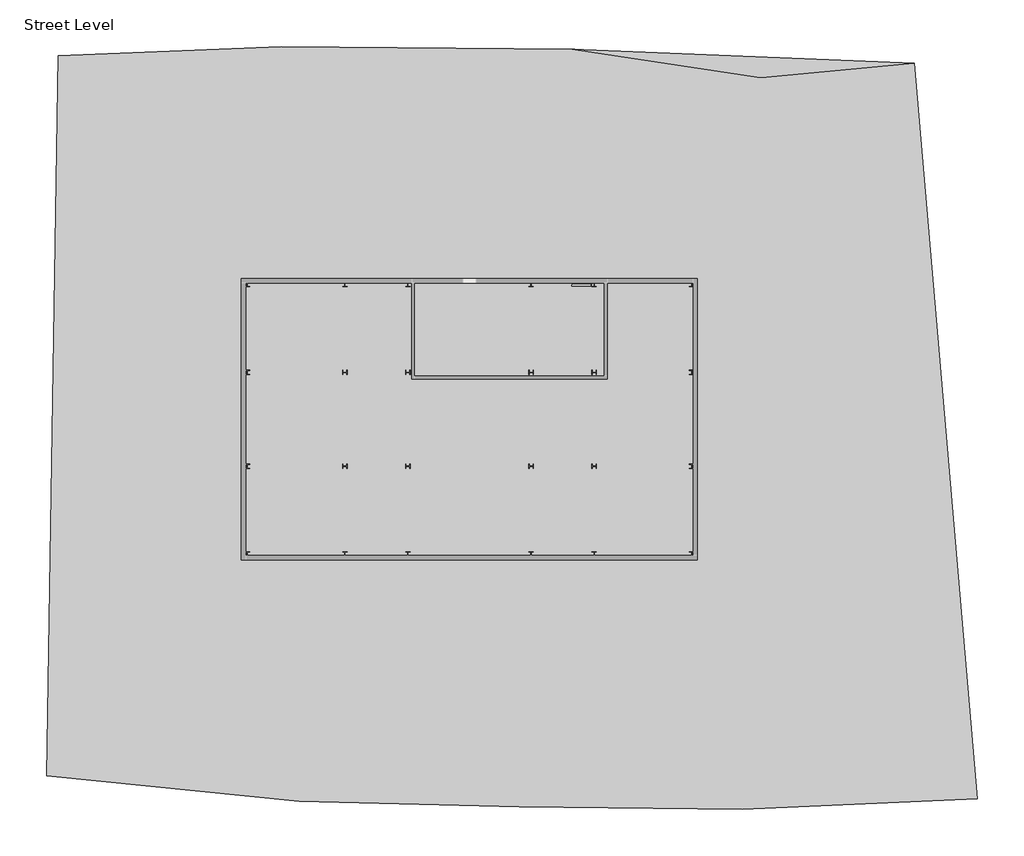
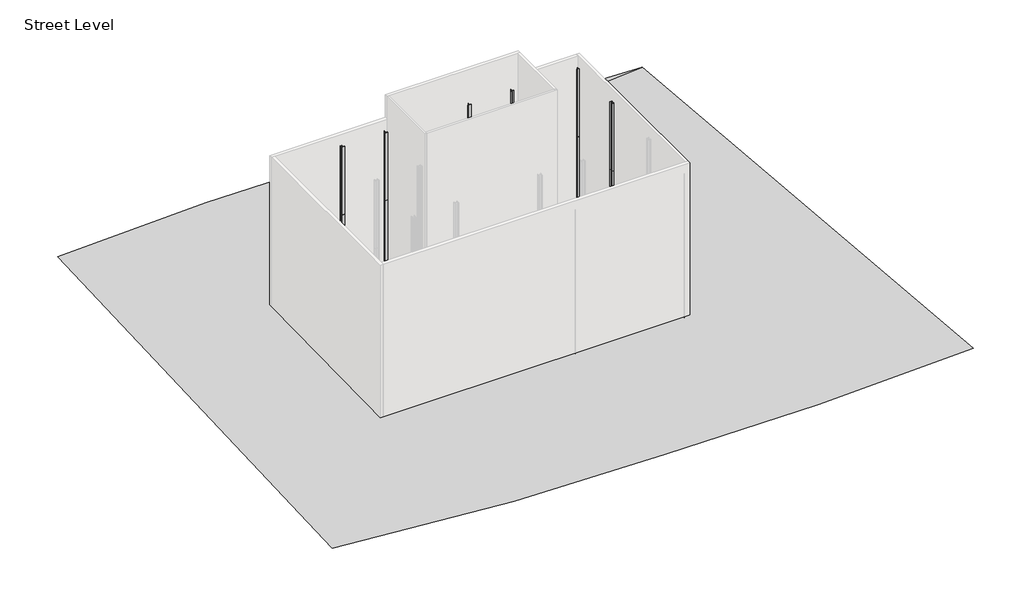
# One storey, part 3 of 3: 8 columns, 1 member, 1 proxy.
"""IFC4 building model written with IfcOpenShell, lengths in millimetres."""

import ifcopenshell
import ifcopenshell.guid

model = None  # the IFC model being written
_history = None  # IfcOwnerHistory: only IFC2X3 demands one
_inside = {}  # id of a spatial element -> (the spatial element, [elements in it])
_under = {}  # id of a project, library or spatial element -> (it, [spatial elements below it])
_declared = {}  # id of a project -> (the project, [libraries it declares])
_typed = {}  # id of a type object -> (the type object, [elements of that type])
_made_of = {}  # id of a material, layer set ... -> (it, [elements and type objects made of it])


def new_model(schema):
    """Start an empty IFC model of exactly this schema.

    Asked for "IFC4X3", IfcOpenShell would pick the latest addendum, in which some entities
    have other attributes; the version numbers below select the first issue.
    IFC2X3 requires an IfcOwnerHistory on every rooted entity: one is made here for all.
    """
    global model, _history
    if schema == "IFC4X3":
        model = ifcopenshell.file(schema_version=(4, 3, 0, 0))
    else:
        model = ifcopenshell.file(schema=schema)
    _inside.clear()
    _under.clear()
    _declared.clear()
    _typed.clear()
    _made_of.clear()
    _history = None
    if model.schema == "IFC2X3":
        org = make("IfcOrganization", Name="unknown")
        user = make(
            "IfcPersonAndOrganization",
            ThePerson=make("IfcPerson", FamilyName="unknown"),
            TheOrganization=org,
        )
        app = make(
            "IfcApplication",
            ApplicationDeveloper=org,
            Version="unknown",
            ApplicationFullName="unknown",
            ApplicationIdentifier="unknown",
        )
        _history = make(
            "IfcOwnerHistory",
            OwningUser=user,
            OwningApplication=app,
            ChangeAction="ADDED",
            CreationDate=0,
        )
    return model


def make(cls, **values):
    """One entity of the class cls with the attributes given. An attribute that is None is left unset."""
    return model.create_entity(
        cls, **{name: value for name, value in values.items() if value is not None}
    )


def rooted(cls, **values):
    """An entity with a GlobalId (a new one), such as an element, a storey or a relation."""
    return make(cls, GlobalId=ifcopenshell.guid.new(), OwnerHistory=_history, **values)


def si_unit(unit_type, name, prefix=None):
    """IfcSIUnit, for example si_unit("LENGTHUNIT", "METRE", prefix="MILLI")."""
    return make("IfcSIUnit", UnitType=unit_type, Prefix=prefix, Name=name)


def assignment(units):
    """IfcUnitAssignment: the units of a project."""
    return None if units is None else make("IfcUnitAssignment", Units=units)


def point(xyz):
    """IfcCartesianPoint."""
    return None if xyz is None else make("IfcCartesianPoint", Coordinates=xyz)


def direction(xyz):
    """IfcDirection."""
    return None if xyz is None else make("IfcDirection", DirectionRatios=xyz)


def frame(location, z_axis=None, x_axis=None):
    """IfcAxis2Placement3D, a coordinate frame: its origin and axes. An axis left out is left unset."""
    return make(
        "IfcAxis2Placement3D",
        Location=point(location),
        Axis=direction(z_axis),
        RefDirection=direction(x_axis),
    )


def frame_2d(location, x_axis=None):
    """IfcAxis2Placement2D, a coordinate frame in the plane: its origin and x axis."""
    return make(
        "IfcAxis2Placement2D", Location=point(location), RefDirection=direction(x_axis)
    )


def origin():
    """The frame at (0, 0, 0) with its axes left unset."""
    return frame((0.0, 0.0, 0.0))


def place(relative_to, where):
    """IfcLocalPlacement: puts the frame where relative to a parent placement (None: the world)."""
    return make(
        "IfcLocalPlacement", PlacementRelTo=relative_to, RelativePlacement=where
    )


def context(
    kind, dimensions, precision=None, world=None, true_north=None, identifier=None
):
    """IfcGeometricRepresentationContext, for example the 3D "Model" context."""
    return make(
        "IfcGeometricRepresentationContext",
        ContextIdentifier=identifier,
        ContextType=kind,
        CoordinateSpaceDimension=dimensions,
        Precision=precision,
        WorldCoordinateSystem=world,
        TrueNorth=true_north,
    )


def project(units=None, contexts=None):
    """IfcProject with its units and contexts."""
    return rooted(
        "IfcProject",
        Name="project",
        RepresentationContexts=contexts,
        UnitsInContext=assignment(units),
    )


def spatial(cls, under=None, at=None, **own):
    """A site, building, storey or space (cls), placed at a placement, below another one or the project."""
    s = rooted(cls, ObjectPlacement=at, **own)
    if under is not None:
        _under.setdefault(under.id(), (under, []))[1].append(s)
    return s


def polyline(points):
    """IfcPolyline through the points."""
    return make("IfcPolyline", Points=[point(p) for p in points])


def point_list(points):
    """IfcCartesianPointList2D or 3D."""
    cls = (
        "IfcCartesianPointList2D" if len(points[0]) == 2 else "IfcCartesianPointList3D"
    )
    return make(cls, CoordList=points)


def circle_curve(where, radius):
    """IfcCircle in the frame where."""
    return make("IfcCircle", Position=where, Radius=radius)


def trimmed(basis, trim1, trim2, sense, master):
    """IfcTrimmedCurve: the piece of a basis curve between two trims."""
    return make(
        "IfcTrimmedCurve",
        BasisCurve=basis,
        Trim1=trim1,
        Trim2=trim2,
        SenseAgreement=sense,
        MasterRepresentation=master,
    )


def segment(curve, same_sense, transition):
    """IfcCompositeCurveSegment."""
    return make(
        "IfcCompositeCurveSegment",
        Transition=transition,
        SameSense=same_sense,
        ParentCurve=curve,
    )


def composite_curve(segments, self_intersect=None):
    """IfcCompositeCurve: segments joined end to end."""
    return make("IfcCompositeCurve", Segments=segments, SelfIntersect=self_intersect)


def outline(outer, holes=None, kind="AREA"):
    """IfcArbitraryClosedProfileDef: a profile drawn as a closed curve; with holes, ...WithVoids."""
    if holes is None:
        return make("IfcArbitraryClosedProfileDef", ProfileType=kind, OuterCurve=outer)
    return make(
        "IfcArbitraryProfileDefWithVoids",
        ProfileType=kind,
        OuterCurve=outer,
        InnerCurves=holes,
    )


def extrude(swept, where, along, depth):
    """IfcExtrudedAreaSolid: the profile swept, set in the frame where, extruded along a direction by depth."""
    return make(
        "IfcExtrudedAreaSolid",
        SweptArea=swept,
        Position=where,
        ExtrudedDirection=direction(along),
        Depth=depth,
    )


def triangles(points, corners, closed=None, point_numbers=None):
    """IfcTriangulatedFaceSet: each triangle names its three corners, points numbered from 1."""
    return make(
        "IfcTriangulatedFaceSet",
        Coordinates=point_list(points),
        Closed=closed,
        CoordIndex=corners,
        PnIndex=point_numbers,
    )


def shape(context_of_items, identifier, shape_type, items):
    """IfcShapeRepresentation: the items that make up one representation, for example the "Body"."""
    return make(
        "IfcShapeRepresentation",
        ContextOfItems=context_of_items,
        RepresentationIdentifier=identifier,
        RepresentationType=shape_type,
        Items=items,
    )


def source(mapping_origin, context_of_items, identifier, shape_type, items):
    """IfcRepresentationMap: a shape defined once, which mapped items show again and again."""
    return make(
        "IfcRepresentationMap",
        MappingOrigin=mapping_origin,
        MappedRepresentation=shape(context_of_items, identifier, shape_type, items),
    )


def transform(
    local_origin,
    x_axis=None,
    y_axis=None,
    z_axis=None,
    scale=None,
    scale2=None,
    scale3=None,
    uniform=True,
):
    """IfcCartesianTransformationOperator3D, or its non-uniform kind. x_axis, y_axis, z_axis: its Axis1, 2, 3."""
    if uniform:
        return make(
            "IfcCartesianTransformationOperator3D",
            Axis1=direction(x_axis),
            Axis2=direction(y_axis),
            LocalOrigin=point(local_origin),
            Scale=scale,
            Axis3=direction(z_axis),
        )
    return make(
        "IfcCartesianTransformationOperator3DnonUniform",
        Axis1=direction(x_axis),
        Axis2=direction(y_axis),
        LocalOrigin=point(local_origin),
        Scale=scale,
        Axis3=direction(z_axis),
        Scale2=scale2,
        Scale3=scale3,
    )


def mapped(mapping_source, mapping_target):
    """IfcMappedItem: shows the shape of a source again, moved by a transform."""
    return make(
        "IfcMappedItem", MappingSource=mapping_source, MappingTarget=mapping_target
    )


def made_of(thing, what):
    """Note that an element or type object is made of a material, layer set ...; save() writes the relation."""
    if what is not None:
        _made_of.setdefault(what.id(), (what, []))[1].append(thing)
    return thing


def element(
    cls,
    number,
    at=None,
    inside=None,
    cuts=None,
    type_object=None,
    material=None,
    context=None,
    identifier="Body",
    shape_type=None,
    held_by="IfcProductDefinitionShape",
    body=None,
    shapes=None,
    **own,
):
    """One element of the class cls, such as IfcWall. Its Tag is "e" and its number.

    at: its placement. inside: the storey or other place that contains it. cuts: it is an
    opening in that element (IfcRelVoidsElement). A single representation is given by context,
    identifier, shape_type and body (its items); several are given by shapes. held_by: the class
    of the entity that holds the representations. save() writes the other relations.
    """
    e = rooted(cls, Tag="e%d" % number, ObjectPlacement=at, **own)
    if body is not None:
        shapes = [shape(context, identifier, shape_type, body)]
    if shapes is not None:
        e.Representation = make(held_by, Representations=shapes)
    if inside is not None:
        _inside.setdefault(inside.id(), (inside, []))[1].append(e)
    if cuts is not None:
        rooted(
            "IfcRelVoidsElement", RelatingBuildingElement=cuts, RelatedOpeningElement=e
        )
    if type_object is not None:
        _typed.setdefault(type_object.id(), (type_object, []))[1].append(e)
    return made_of(e, material)


def aggregate(whole, parts):
    """IfcRelAggregates: a whole, such as a stair, and the parts it consists of."""
    return rooted("IfcRelAggregates", RelatingObject=whole, RelatedObjects=parts)


def save(model, path):
    """Write the relations noted so far, then the file.

    IfcRelAggregates (storeys below a building ...), IfcRelContainedInSpatialStructure (elements
    in a storey), IfcRelDefinesByType, IfcRelAssociatesMaterial and IfcRelDeclares: one each for
    every whole, place, type object, material and project.
    """
    for whole, parts in _under.values():
        aggregate(whole, parts)
    for where, things in _inside.values():
        rooted(
            "IfcRelContainedInSpatialStructure",
            RelatedElements=things,
            RelatingStructure=where,
        )
    for kind, things in _typed.values():
        rooted("IfcRelDefinesByType", RelatedObjects=things, RelatingType=kind)
    for what, things in _made_of.values():
        rooted("IfcRelAssociatesMaterial", RelatedObjects=things, RelatingMaterial=what)
    for by, libraries in _declared.values():
        rooted("IfcRelDeclares", RelatingContext=by, RelatedDefinitions=libraries)
    model.write(path)


def l_angle_l6x6x3_8_1e5b70da(model_context):
    return source(origin(), model_context, "Body", "SweptSolid", [
        extrude(outline(composite_curve([segment(polyline([(41.148, 41.148), (41.148, -111.252)]), True, "CONTINUOUS"), segment(trimmed(circle_curve(frame_2d((41.148, -101.727)), 9.525), [point((41.148, -111.252))], [point((31.623, -101.727))], False, "CARTESIAN"), True, "CONTINUOUS"), segment(polyline([(31.623, -101.727), (31.623, 22.098)]), True, "CONTINUOUS"), segment(trimmed(circle_curve(frame_2d((22.098, 22.098)), 9.525), [point((31.623, 22.098))], [point((22.098, 31.623))], True, "CARTESIAN"), True, "CONTINUOUS"), segment(polyline([(22.098, 31.623), (-101.727, 31.623)]), True, "CONTINUOUS"), segment(trimmed(circle_curve(frame_2d((-101.727, 41.148)), 9.525), [point((-101.727, 31.623))], [point((-111.252, 41.148))], False, "CARTESIAN"), True, "CONTINUOUS"), segment(polyline([(-111.252, 41.148), (41.148, 41.148)]), True, "CONTINUOUS")], self_intersect=False)), frame((-2053.4214347, 0.0, 0.0), z_axis=(1.0, 0.0, 0.0), x_axis=(0.0, 1.0, 0.0)), (0.0, 0.0, 1.0), 4092.1699392),
    ])


model = new_model("IFC4")

# Units and contexts
model_context = context("Model", 3, world=origin())
ifc_project = project(units=[si_unit("LENGTHUNIT", "METRE", prefix="MILLI")], contexts=[model_context])

# Site, building, storey
site = spatial("IfcSite", under=ifc_project)
building = spatial("IfcBuilding", under=site)
storey = spatial("IfcBuildingStorey", under=building, Name="Street Level", Elevation=-914.4)

# Proxy
placement = place(None, origin())
element("IfcBuildingElementProxy", 1, Name="Building Element Proxy", at=placement, inside=storey, context=model_context, shape_type="Tessellation", body=[
    triangles([(-29664.1428223, 25063.2445862, 0.0), (-14195.9393097, 25689.5644958, 0.0), (5935.7725708, 25510.6149536, 0.0), (18999.0170654, 23542.1816162, 0.0), (29646.4555298, 24526.3982849, 0.0), (-30469.4122742, -24863.4009705, -914.4), (-12943.2994904, -26652.8870911, -914.4), (2267.3273026, -27010.7838501, -914.4), (17746.3772461, -27189.7333923, -914.4), (34030.6948975, -26473.9375488, -914.4)], [[7, 8, 2], [6, 2, 1], [2, 6, 7], [8, 3, 2], [9, 10, 4], [3, 4, 5], [3, 8, 4], [5, 4, 10], [4, 8, 9]], closed=False),
])

# Columns
element("IfcColumn", 2, ObjectType="W-Wide Flange-Column : W12X87", at=placement, inside=storey, context=model_context, shape_type="SweptSolid", body=[
    extrude(outline(composite_curve([segment(polyline([(3260.1377268, 2940.2315304), (3239.5637268, 2940.2315304), (3239.5637268, 3065.0725304)]), True, "CONTINUOUS"), segment(trimmed(circle_curve(frame_2d((3217.2752268, 3065.0725304)), 22.2885), [point((3239.5637268, 3065.0725304))], [point((3217.2752268, 3087.3610304))], True, "CARTESIAN"), True, "CONTINUOUS"), segment(polyline([(3217.2752268, 3087.3610304), (2985.5002268, 3087.3610304)]), True, "CONTINUOUS"), segment(trimmed(circle_curve(frame_2d((2985.5002268, 3065.0725304)), 22.2885), [point((2985.5002268, 3087.3610304))], [point((2963.2117268, 3065.0725304))], True, "CARTESIAN"), True, "CONTINUOUS"), segment(polyline([(2963.2117268, 3065.0725304), (2963.2117268, 2940.2315304), (2942.6377268, 2940.2315304), (2942.6377268, 3247.5715304), (2963.2117268, 3247.5715304), (2963.2117268, 3122.7305304)]), True, "CONTINUOUS"), segment(trimmed(circle_curve(frame_2d((2985.5002268, 3122.7305304)), 22.2885), [point((2963.2117268, 3122.7305304))], [point((2985.5002268, 3100.4420304))], True, "CARTESIAN"), True, "CONTINUOUS"), segment(polyline([(2985.5002268, 3100.4420304), (3217.2752268, 3100.4420304)]), True, "CONTINUOUS"), segment(trimmed(circle_curve(frame_2d((3217.2752268, 3122.7305304)), 22.2885), [point((3217.2752268, 3100.4420304))], [point((3239.5637268, 3122.7305304))], True, "CARTESIAN"), True, "CONTINUOUS"), segment(polyline([(3239.5637268, 3122.7305304), (3239.5637268, 3247.5715304), (3260.1377268, 3247.5715304), (3260.1377268, 2940.2315304)]), True, "CONTINUOUS")], self_intersect=False)), frame((0.0, 0.0, 7315.2), z_axis=(0.0, 0.0, 1.0), x_axis=(1.0, 0.0, 0.0)), (0.0, 0.0, 1.0), 7315.2),
    extrude(outline(composite_curve([segment(polyline([(3260.1377268, 2940.2315304), (3239.5637268, 2940.2315304), (3239.5637268, 3065.0725304)]), True, "CONTINUOUS"), segment(trimmed(circle_curve(frame_2d((3217.2752268, 3065.0725304)), 22.2885), [point((3239.5637268, 3065.0725304))], [point((3217.2752268, 3087.3610304))], True, "CARTESIAN"), True, "CONTINUOUS"), segment(polyline([(3217.2752268, 3087.3610304), (2985.5002268, 3087.3610304)]), True, "CONTINUOUS"), segment(trimmed(circle_curve(frame_2d((2985.5002268, 3065.0725304)), 22.2885), [point((2985.5002268, 3087.3610304))], [point((2963.2117268, 3065.0725304))], True, "CARTESIAN"), True, "CONTINUOUS"), segment(polyline([(2963.2117268, 3065.0725304), (2963.2117268, 2940.2315304), (2942.6377268, 2940.2315304), (2942.6377268, 3247.5715304), (2963.2117268, 3247.5715304), (2963.2117268, 3122.7305304)]), True, "CONTINUOUS"), segment(trimmed(circle_curve(frame_2d((2985.5002268, 3122.7305304)), 22.2885), [point((2963.2117268, 3122.7305304))], [point((2985.5002268, 3100.4420304))], True, "CARTESIAN"), True, "CONTINUOUS"), segment(polyline([(2985.5002268, 3100.4420304), (3217.2752268, 3100.4420304)]), True, "CONTINUOUS"), segment(trimmed(circle_curve(frame_2d((3217.2752268, 3122.7305304)), 22.2885), [point((3217.2752268, 3100.4420304))], [point((3239.5637268, 3122.7305304))], True, "CARTESIAN"), True, "CONTINUOUS"), segment(polyline([(3239.5637268, 3122.7305304), (3239.5637268, 3247.5715304), (3260.1377268, 3247.5715304), (3260.1377268, 2940.2315304)]), True, "CONTINUOUS")], self_intersect=False)), frame((0.0, 0.0, -914.4), z_axis=(0.0, 0.0, 1.0), x_axis=(1.0, 0.0, 0.0)), (0.0, 0.0, 1.0), 8229.6),
])
element("IfcColumn", 3, ObjectType="W-Wide Flange-Column : W12X87", at=placement, inside=storey, context=model_context, shape_type="SweptSolid", body=[
    extrude(outline(composite_curve([segment(polyline([(7628.9377268, 2940.2315304), (7608.3637268, 2940.2315304), (7608.3637268, 3065.0725304)]), True, "CONTINUOUS"), segment(trimmed(circle_curve(frame_2d((7586.0752268, 3065.0725304)), 22.2885), [point((7608.3637268, 3065.0725304))], [point((7586.0752268, 3087.3610304))], True, "CARTESIAN"), True, "CONTINUOUS"), segment(polyline([(7586.0752268, 3087.3610304), (7354.3002268, 3087.3610304)]), True, "CONTINUOUS"), segment(trimmed(circle_curve(frame_2d((7354.3002268, 3065.0725304)), 22.2885), [point((7354.3002268, 3087.3610304))], [point((7332.0117268, 3065.0725304))], True, "CARTESIAN"), True, "CONTINUOUS"), segment(polyline([(7332.0117268, 3065.0725304), (7332.0117268, 2940.2315304), (7311.4377268, 2940.2315304), (7311.4377268, 3247.5715304), (7332.0117268, 3247.5715304), (7332.0117268, 3122.7305304)]), True, "CONTINUOUS"), segment(trimmed(circle_curve(frame_2d((7354.3002268, 3122.7305304)), 22.2885), [point((7332.0117268, 3122.7305304))], [point((7354.3002268, 3100.4420304))], True, "CARTESIAN"), True, "CONTINUOUS"), segment(polyline([(7354.3002268, 3100.4420304), (7586.0752268, 3100.4420304)]), True, "CONTINUOUS"), segment(trimmed(circle_curve(frame_2d((7586.0752268, 3122.7305304)), 22.2885), [point((7586.0752268, 3100.4420304))], [point((7608.3637268, 3122.7305304))], True, "CARTESIAN"), True, "CONTINUOUS"), segment(polyline([(7608.3637268, 3122.7305304), (7608.3637268, 3247.5715304), (7628.9377268, 3247.5715304), (7628.9377268, 2940.2315304)]), True, "CONTINUOUS")], self_intersect=False)), frame((0.0, 0.0, 7315.2), z_axis=(0.0, 0.0, 1.0), x_axis=(1.0, 0.0, 0.0)), (0.0, 0.0, 1.0), 7315.2),
    extrude(outline(composite_curve([segment(polyline([(7628.9377268, 2940.2315304), (7608.3637268, 2940.2315304), (7608.3637268, 3065.0725304)]), True, "CONTINUOUS"), segment(trimmed(circle_curve(frame_2d((7586.0752268, 3065.0725304)), 22.2885), [point((7608.3637268, 3065.0725304))], [point((7586.0752268, 3087.3610304))], True, "CARTESIAN"), True, "CONTINUOUS"), segment(polyline([(7586.0752268, 3087.3610304), (7354.3002268, 3087.3610304)]), True, "CONTINUOUS"), segment(trimmed(circle_curve(frame_2d((7354.3002268, 3065.0725304)), 22.2885), [point((7354.3002268, 3087.3610304))], [point((7332.0117268, 3065.0725304))], True, "CARTESIAN"), True, "CONTINUOUS"), segment(polyline([(7332.0117268, 3065.0725304), (7332.0117268, 2940.2315304), (7311.4377268, 2940.2315304), (7311.4377268, 3247.5715304), (7332.0117268, 3247.5715304), (7332.0117268, 3122.7305304)]), True, "CONTINUOUS"), segment(trimmed(circle_curve(frame_2d((7354.3002268, 3122.7305304)), 22.2885), [point((7332.0117268, 3122.7305304))], [point((7354.3002268, 3100.4420304))], True, "CARTESIAN"), True, "CONTINUOUS"), segment(polyline([(7354.3002268, 3100.4420304), (7586.0752268, 3100.4420304)]), True, "CONTINUOUS"), segment(trimmed(circle_curve(frame_2d((7586.0752268, 3122.7305304)), 22.2885), [point((7586.0752268, 3100.4420304))], [point((7608.3637268, 3122.7305304))], True, "CARTESIAN"), True, "CONTINUOUS"), segment(polyline([(7608.3637268, 3122.7305304), (7608.3637268, 3247.5715304), (7628.9377268, 3247.5715304), (7628.9377268, 2940.2315304)]), True, "CONTINUOUS")], self_intersect=False)), frame((0.0, 0.0, -914.4), z_axis=(0.0, 0.0, 1.0), x_axis=(1.0, 0.0, 0.0)), (0.0, 0.0, 1.0), 8229.6),
])
element("IfcColumn", 4, ObjectType="W-Wide Flange-Column : W12X87", at=placement, inside=storey, context=model_context, shape_type="SweptSolid", body=[
    extrude(outline(composite_curve([segment(polyline([(-9648.1422732, 9348.6515304), (-9648.1422732, 9328.0775304), (-9772.9832732, 9328.0775304)]), True, "CONTINUOUS"), segment(trimmed(circle_curve(frame_2d((-9772.9832732, 9305.7890304)), 22.2885), [point((-9772.9832732, 9328.0775304))], [point((-9795.2717732, 9305.7890304))], True, "CARTESIAN"), True, "CONTINUOUS"), segment(polyline([(-9795.2717732, 9305.7890304), (-9795.2717732, 9074.0140304)]), True, "CONTINUOUS"), segment(trimmed(circle_curve(frame_2d((-9772.9832732, 9074.0140304)), 22.2885), [point((-9795.2717732, 9074.0140304))], [point((-9772.9832732, 9051.7255304))], True, "CARTESIAN"), True, "CONTINUOUS"), segment(polyline([(-9772.9832732, 9051.7255304), (-9648.1422732, 9051.7255304), (-9648.1422732, 9031.1515304), (-9955.4822732, 9031.1515304), (-9955.4822732, 9051.7255304), (-9830.6412732, 9051.7255304)]), True, "CONTINUOUS"), segment(trimmed(circle_curve(frame_2d((-9830.6412732, 9074.0140304)), 22.2885), [point((-9830.6412732, 9051.7255304))], [point((-9808.3527732, 9074.0140304))], True, "CARTESIAN"), True, "CONTINUOUS"), segment(polyline([(-9808.3527732, 9074.0140304), (-9808.3527732, 9305.7890304)]), True, "CONTINUOUS"), segment(trimmed(circle_curve(frame_2d((-9830.6412732, 9305.7890304)), 22.2885), [point((-9808.3527732, 9305.7890304))], [point((-9830.6412732, 9328.0775304))], True, "CARTESIAN"), True, "CONTINUOUS"), segment(polyline([(-9830.6412732, 9328.0775304), (-9955.4822732, 9328.0775304), (-9955.4822732, 9348.6515304), (-9648.1422732, 9348.6515304)]), True, "CONTINUOUS")], self_intersect=False)), frame((0.0, 0.0, 7315.2), z_axis=(0.0, 0.0, 1.0), x_axis=(1.0, 0.0, 0.0)), (0.0, 0.0, 1.0), 7315.2),
    extrude(outline(composite_curve([segment(polyline([(-9648.1422732, 9348.6515304), (-9648.1422732, 9328.0775304), (-9772.9832732, 9328.0775304)]), True, "CONTINUOUS"), segment(trimmed(circle_curve(frame_2d((-9772.9832732, 9305.7890304)), 22.2885), [point((-9772.9832732, 9328.0775304))], [point((-9795.2717732, 9305.7890304))], True, "CARTESIAN"), True, "CONTINUOUS"), segment(polyline([(-9795.2717732, 9305.7890304), (-9795.2717732, 9074.0140304)]), True, "CONTINUOUS"), segment(trimmed(circle_curve(frame_2d((-9772.9832732, 9074.0140304)), 22.2885), [point((-9795.2717732, 9074.0140304))], [point((-9772.9832732, 9051.7255304))], True, "CARTESIAN"), True, "CONTINUOUS"), segment(polyline([(-9772.9832732, 9051.7255304), (-9648.1422732, 9051.7255304), (-9648.1422732, 9031.1515304), (-9955.4822732, 9031.1515304), (-9955.4822732, 9051.7255304), (-9830.6412732, 9051.7255304)]), True, "CONTINUOUS"), segment(trimmed(circle_curve(frame_2d((-9830.6412732, 9074.0140304)), 22.2885), [point((-9830.6412732, 9051.7255304))], [point((-9808.3527732, 9074.0140304))], True, "CARTESIAN"), True, "CONTINUOUS"), segment(polyline([(-9808.3527732, 9074.0140304), (-9808.3527732, 9305.7890304)]), True, "CONTINUOUS"), segment(trimmed(circle_curve(frame_2d((-9830.6412732, 9305.7890304)), 22.2885), [point((-9808.3527732, 9305.7890304))], [point((-9830.6412732, 9328.0775304))], True, "CARTESIAN"), True, "CONTINUOUS"), segment(polyline([(-9830.6412732, 9328.0775304), (-9955.4822732, 9328.0775304), (-9955.4822732, 9348.6515304), (-9648.1422732, 9348.6515304)]), True, "CONTINUOUS")], self_intersect=False)), frame((0.0, 0.0, -914.4), z_axis=(0.0, 0.0, 1.0), x_axis=(1.0, 0.0, 0.0)), (0.0, 0.0, 1.0), 8229.6),
])
element("IfcColumn", 5, ObjectType="W-Wide Flange-Column : W12X87", at=placement, inside=storey, context=model_context, shape_type="SweptSolid", body=[
    extrude(outline(composite_curve([segment(polyline([(-5279.3422732, 9348.6515304), (-5279.3422732, 9328.0775304), (-5404.1832732, 9328.0775304)]), True, "CONTINUOUS"), segment(trimmed(circle_curve(frame_2d((-5404.1832732, 9305.7890304)), 22.2885), [point((-5404.1832732, 9328.0775304))], [point((-5426.4717732, 9305.7890304))], True, "CARTESIAN"), True, "CONTINUOUS"), segment(polyline([(-5426.4717732, 9305.7890304), (-5426.4717732, 9074.0140304)]), True, "CONTINUOUS"), segment(trimmed(circle_curve(frame_2d((-5404.1832732, 9074.0140304)), 22.2885), [point((-5426.4717732, 9074.0140304))], [point((-5404.1832732, 9051.7255304))], True, "CARTESIAN"), True, "CONTINUOUS"), segment(polyline([(-5404.1832732, 9051.7255304), (-5279.3422732, 9051.7255304), (-5279.3422732, 9031.1515304), (-5586.6822732, 9031.1515304), (-5586.6822732, 9051.7255304), (-5461.8412732, 9051.7255304)]), True, "CONTINUOUS"), segment(trimmed(circle_curve(frame_2d((-5461.8412732, 9074.0140304)), 22.2885), [point((-5461.8412732, 9051.7255304))], [point((-5439.5527732, 9074.0140304))], True, "CARTESIAN"), True, "CONTINUOUS"), segment(polyline([(-5439.5527732, 9074.0140304), (-5439.5527732, 9305.7890304)]), True, "CONTINUOUS"), segment(trimmed(circle_curve(frame_2d((-5461.8412732, 9305.7890304)), 22.2885), [point((-5439.5527732, 9305.7890304))], [point((-5461.8412732, 9328.0775304))], True, "CARTESIAN"), True, "CONTINUOUS"), segment(polyline([(-5461.8412732, 9328.0775304), (-5586.6822732, 9328.0775304), (-5586.6822732, 9348.6515304), (-5279.3422732, 9348.6515304)]), True, "CONTINUOUS")], self_intersect=False)), frame((0.0, 0.0, 7315.2), z_axis=(0.0, 0.0, 1.0), x_axis=(1.0, 0.0, 0.0)), (0.0, 0.0, 1.0), 7315.2),
    extrude(outline(composite_curve([segment(polyline([(-5279.3422732, 9348.6515304), (-5279.3422732, 9328.0775304), (-5404.1832732, 9328.0775304)]), True, "CONTINUOUS"), segment(trimmed(circle_curve(frame_2d((-5404.1832732, 9305.7890304)), 22.2885), [point((-5404.1832732, 9328.0775304))], [point((-5426.4717732, 9305.7890304))], True, "CARTESIAN"), True, "CONTINUOUS"), segment(polyline([(-5426.4717732, 9305.7890304), (-5426.4717732, 9074.0140304)]), True, "CONTINUOUS"), segment(trimmed(circle_curve(frame_2d((-5404.1832732, 9074.0140304)), 22.2885), [point((-5426.4717732, 9074.0140304))], [point((-5404.1832732, 9051.7255304))], True, "CARTESIAN"), True, "CONTINUOUS"), segment(polyline([(-5404.1832732, 9051.7255304), (-5279.3422732, 9051.7255304), (-5279.3422732, 9031.1515304), (-5586.6822732, 9031.1515304), (-5586.6822732, 9051.7255304), (-5461.8412732, 9051.7255304)]), True, "CONTINUOUS"), segment(trimmed(circle_curve(frame_2d((-5461.8412732, 9074.0140304)), 22.2885), [point((-5461.8412732, 9051.7255304))], [point((-5439.5527732, 9074.0140304))], True, "CARTESIAN"), True, "CONTINUOUS"), segment(polyline([(-5439.5527732, 9074.0140304), (-5439.5527732, 9305.7890304)]), True, "CONTINUOUS"), segment(trimmed(circle_curve(frame_2d((-5461.8412732, 9305.7890304)), 22.2885), [point((-5439.5527732, 9305.7890304))], [point((-5461.8412732, 9328.0775304))], True, "CARTESIAN"), True, "CONTINUOUS"), segment(polyline([(-5461.8412732, 9328.0775304), (-5586.6822732, 9328.0775304), (-5586.6822732, 9348.6515304), (-5279.3422732, 9348.6515304)]), True, "CONTINUOUS")], self_intersect=False)), frame((0.0, 0.0, -914.4), z_axis=(0.0, 0.0, 1.0), x_axis=(1.0, 0.0, 0.0)), (0.0, 0.0, 1.0), 8229.6),
])
element("IfcColumn", 6, ObjectType="W-Wide Flange-Column : W12X87", at=placement, inside=storey, context=model_context, shape_type="SweptSolid", body=[
    extrude(outline(composite_curve([segment(polyline([(3255.0577268, 9348.6515304), (3255.0577268, 9328.0775304), (3130.2167268, 9328.0775304)]), True, "CONTINUOUS"), segment(trimmed(circle_curve(frame_2d((3130.2167268, 9305.7890304)), 22.2885), [point((3130.2167268, 9328.0775304))], [point((3107.9282268, 9305.7890304))], True, "CARTESIAN"), True, "CONTINUOUS"), segment(polyline([(3107.9282268, 9305.7890304), (3107.9282268, 9074.0140304)]), True, "CONTINUOUS"), segment(trimmed(circle_curve(frame_2d((3130.2167268, 9074.0140304)), 22.2885), [point((3107.9282268, 9074.0140304))], [point((3130.2167268, 9051.7255304))], True, "CARTESIAN"), True, "CONTINUOUS"), segment(polyline([(3130.2167268, 9051.7255304), (3255.0577268, 9051.7255304), (3255.0577268, 9031.1515304), (2947.7177268, 9031.1515304), (2947.7177268, 9051.7255304), (3072.5587268, 9051.7255304)]), True, "CONTINUOUS"), segment(trimmed(circle_curve(frame_2d((3072.5587268, 9074.0140304)), 22.2885), [point((3072.5587268, 9051.7255304))], [point((3094.8472268, 9074.0140304))], True, "CARTESIAN"), True, "CONTINUOUS"), segment(polyline([(3094.8472268, 9074.0140304), (3094.8472268, 9305.7890304)]), True, "CONTINUOUS"), segment(trimmed(circle_curve(frame_2d((3072.5587268, 9305.7890304)), 22.2885), [point((3094.8472268, 9305.7890304))], [point((3072.5587268, 9328.0775304))], True, "CARTESIAN"), True, "CONTINUOUS"), segment(polyline([(3072.5587268, 9328.0775304), (2947.7177268, 9328.0775304), (2947.7177268, 9348.6515304), (3255.0577268, 9348.6515304)]), True, "CONTINUOUS")], self_intersect=False)), frame((0.0, 0.0, 7315.2), z_axis=(0.0, 0.0, 1.0), x_axis=(1.0, 0.0, 0.0)), (0.0, 0.0, 1.0), 7315.2),
    extrude(outline(composite_curve([segment(polyline([(3255.0577268, 9348.6515304), (3255.0577268, 9328.0775304), (3130.2167268, 9328.0775304)]), True, "CONTINUOUS"), segment(trimmed(circle_curve(frame_2d((3130.2167268, 9305.7890304)), 22.2885), [point((3130.2167268, 9328.0775304))], [point((3107.9282268, 9305.7890304))], True, "CARTESIAN"), True, "CONTINUOUS"), segment(polyline([(3107.9282268, 9305.7890304), (3107.9282268, 9074.0140304)]), True, "CONTINUOUS"), segment(trimmed(circle_curve(frame_2d((3130.2167268, 9074.0140304)), 22.2885), [point((3107.9282268, 9074.0140304))], [point((3130.2167268, 9051.7255304))], True, "CARTESIAN"), True, "CONTINUOUS"), segment(polyline([(3130.2167268, 9051.7255304), (3255.0577268, 9051.7255304), (3255.0577268, 9031.1515304), (2947.7177268, 9031.1515304), (2947.7177268, 9051.7255304), (3072.5587268, 9051.7255304)]), True, "CONTINUOUS"), segment(trimmed(circle_curve(frame_2d((3072.5587268, 9074.0140304)), 22.2885), [point((3072.5587268, 9051.7255304))], [point((3094.8472268, 9074.0140304))], True, "CARTESIAN"), True, "CONTINUOUS"), segment(polyline([(3094.8472268, 9074.0140304), (3094.8472268, 9305.7890304)]), True, "CONTINUOUS"), segment(trimmed(circle_curve(frame_2d((3072.5587268, 9305.7890304)), 22.2885), [point((3094.8472268, 9305.7890304))], [point((3072.5587268, 9328.0775304))], True, "CARTESIAN"), True, "CONTINUOUS"), segment(polyline([(3072.5587268, 9328.0775304), (2947.7177268, 9328.0775304), (2947.7177268, 9348.6515304), (3255.0577268, 9348.6515304)]), True, "CONTINUOUS")], self_intersect=False)), frame((0.0, 0.0, -914.4), z_axis=(0.0, 0.0, 1.0), x_axis=(1.0, 0.0, 0.0)), (0.0, 0.0, 1.0), 8229.6),
])
element("IfcColumn", 7, ObjectType="W-Wide Flange-Column : W12X87", at=placement, inside=storey, context=model_context, shape_type="SweptSolid", body=[
    extrude(outline(composite_curve([segment(polyline([(7623.8577268, 9348.6515304), (7623.8577268, 9328.0775304), (7499.0167268, 9328.0775304)]), True, "CONTINUOUS"), segment(trimmed(circle_curve(frame_2d((7499.0167268, 9305.7890304)), 22.2885), [point((7499.0167268, 9328.0775304))], [point((7476.7282268, 9305.7890304))], True, "CARTESIAN"), True, "CONTINUOUS"), segment(polyline([(7476.7282268, 9305.7890304), (7476.7282268, 9074.0140304)]), True, "CONTINUOUS"), segment(trimmed(circle_curve(frame_2d((7499.0167268, 9074.0140304)), 22.2885), [point((7476.7282268, 9074.0140304))], [point((7499.0167268, 9051.7255304))], True, "CARTESIAN"), True, "CONTINUOUS"), segment(polyline([(7499.0167268, 9051.7255304), (7623.8577268, 9051.7255304), (7623.8577268, 9031.1515304), (7316.5177268, 9031.1515304), (7316.5177268, 9051.7255304), (7441.3587268, 9051.7255304)]), True, "CONTINUOUS"), segment(trimmed(circle_curve(frame_2d((7441.3587268, 9074.0140304)), 22.2885), [point((7441.3587268, 9051.7255304))], [point((7463.6472268, 9074.0140304))], True, "CARTESIAN"), True, "CONTINUOUS"), segment(polyline([(7463.6472268, 9074.0140304), (7463.6472268, 9305.7890304)]), True, "CONTINUOUS"), segment(trimmed(circle_curve(frame_2d((7441.3587268, 9305.7890304)), 22.2885), [point((7463.6472268, 9305.7890304))], [point((7441.3587268, 9328.0775304))], True, "CARTESIAN"), True, "CONTINUOUS"), segment(polyline([(7441.3587268, 9328.0775304), (7316.5177268, 9328.0775304), (7316.5177268, 9348.6515304), (7623.8577268, 9348.6515304)]), True, "CONTINUOUS")], self_intersect=False)), frame((0.0, 0.0, 7315.2), z_axis=(0.0, 0.0, 1.0), x_axis=(1.0, 0.0, 0.0)), (0.0, 0.0, 1.0), 7315.2),
    extrude(outline(composite_curve([segment(polyline([(7623.8577268, 9348.6515304), (7623.8577268, 9328.0775304), (7499.0167268, 9328.0775304)]), True, "CONTINUOUS"), segment(trimmed(circle_curve(frame_2d((7499.0167268, 9305.7890304)), 22.2885), [point((7499.0167268, 9328.0775304))], [point((7476.7282268, 9305.7890304))], True, "CARTESIAN"), True, "CONTINUOUS"), segment(polyline([(7476.7282268, 9305.7890304), (7476.7282268, 9074.0140304)]), True, "CONTINUOUS"), segment(trimmed(circle_curve(frame_2d((7499.0167268, 9074.0140304)), 22.2885), [point((7476.7282268, 9074.0140304))], [point((7499.0167268, 9051.7255304))], True, "CARTESIAN"), True, "CONTINUOUS"), segment(polyline([(7499.0167268, 9051.7255304), (7623.8577268, 9051.7255304), (7623.8577268, 9031.1515304), (7316.5177268, 9031.1515304), (7316.5177268, 9051.7255304), (7441.3587268, 9051.7255304)]), True, "CONTINUOUS"), segment(trimmed(circle_curve(frame_2d((7441.3587268, 9074.0140304)), 22.2885), [point((7441.3587268, 9051.7255304))], [point((7463.6472268, 9074.0140304))], True, "CARTESIAN"), True, "CONTINUOUS"), segment(polyline([(7463.6472268, 9074.0140304), (7463.6472268, 9305.7890304)]), True, "CONTINUOUS"), segment(trimmed(circle_curve(frame_2d((7441.3587268, 9305.7890304)), 22.2885), [point((7463.6472268, 9305.7890304))], [point((7441.3587268, 9328.0775304))], True, "CARTESIAN"), True, "CONTINUOUS"), segment(polyline([(7441.3587268, 9328.0775304), (7316.5177268, 9328.0775304), (7316.5177268, 9348.6515304), (7623.8577268, 9348.6515304)]), True, "CONTINUOUS")], self_intersect=False)), frame((0.0, 0.0, -914.4), z_axis=(0.0, 0.0, 1.0), x_axis=(1.0, 0.0, 0.0)), (0.0, 0.0, 1.0), 8229.6),
])
element("IfcColumn", 8, ObjectType="W-Wide Flange-Column : W12X87", at=placement, inside=storey, context=model_context, shape_type="SweptSolid", body=[
    extrude(outline(composite_curve([segment(polyline([(14380.2577268, 9348.6515304), (14380.2577268, 9328.0775304), (14255.4167268, 9328.0775304)]), True, "CONTINUOUS"), segment(trimmed(circle_curve(frame_2d((14255.4167268, 9305.7890304)), 22.2885), [point((14255.4167268, 9328.0775304))], [point((14233.1282268, 9305.7890304))], True, "CARTESIAN"), True, "CONTINUOUS"), segment(polyline([(14233.1282268, 9305.7890304), (14233.1282268, 9074.0140304)]), True, "CONTINUOUS"), segment(trimmed(circle_curve(frame_2d((14255.4167268, 9074.0140304)), 22.2885), [point((14233.1282268, 9074.0140304))], [point((14255.4167268, 9051.7255304))], True, "CARTESIAN"), True, "CONTINUOUS"), segment(polyline([(14255.4167268, 9051.7255304), (14380.2577268, 9051.7255304), (14380.2577268, 9031.1515304), (14072.9177268, 9031.1515304), (14072.9177268, 9051.7255304), (14197.7587268, 9051.7255304)]), True, "CONTINUOUS"), segment(trimmed(circle_curve(frame_2d((14197.7587268, 9074.0140304)), 22.2885), [point((14197.7587268, 9051.7255304))], [point((14220.0472268, 9074.0140304))], True, "CARTESIAN"), True, "CONTINUOUS"), segment(polyline([(14220.0472268, 9074.0140304), (14220.0472268, 9305.7890304)]), True, "CONTINUOUS"), segment(trimmed(circle_curve(frame_2d((14197.7587268, 9305.7890304)), 22.2885), [point((14220.0472268, 9305.7890304))], [point((14197.7587268, 9328.0775304))], True, "CARTESIAN"), True, "CONTINUOUS"), segment(polyline([(14197.7587268, 9328.0775304), (14072.9177268, 9328.0775304), (14072.9177268, 9348.6515304), (14380.2577268, 9348.6515304)]), True, "CONTINUOUS")], self_intersect=False)), frame((0.0, 0.0, 7315.2), z_axis=(0.0, 0.0, 1.0), x_axis=(1.0, 0.0, 0.0)), (0.0, 0.0, 1.0), 7315.2),
    extrude(outline(composite_curve([segment(polyline([(14380.2577268, 9348.6515304), (14380.2577268, 9328.0775304), (14255.4167268, 9328.0775304)]), True, "CONTINUOUS"), segment(trimmed(circle_curve(frame_2d((14255.4167268, 9305.7890304)), 22.2885), [point((14255.4167268, 9328.0775304))], [point((14233.1282268, 9305.7890304))], True, "CARTESIAN"), True, "CONTINUOUS"), segment(polyline([(14233.1282268, 9305.7890304), (14233.1282268, 9074.0140304)]), True, "CONTINUOUS"), segment(trimmed(circle_curve(frame_2d((14255.4167268, 9074.0140304)), 22.2885), [point((14233.1282268, 9074.0140304))], [point((14255.4167268, 9051.7255304))], True, "CARTESIAN"), True, "CONTINUOUS"), segment(polyline([(14255.4167268, 9051.7255304), (14380.2577268, 9051.7255304), (14380.2577268, 9031.1515304), (14072.9177268, 9031.1515304), (14072.9177268, 9051.7255304), (14197.7587268, 9051.7255304)]), True, "CONTINUOUS"), segment(trimmed(circle_curve(frame_2d((14197.7587268, 9074.0140304)), 22.2885), [point((14197.7587268, 9051.7255304))], [point((14220.0472268, 9074.0140304))], True, "CARTESIAN"), True, "CONTINUOUS"), segment(polyline([(14220.0472268, 9074.0140304), (14220.0472268, 9305.7890304)]), True, "CONTINUOUS"), segment(trimmed(circle_curve(frame_2d((14197.7587268, 9305.7890304)), 22.2885), [point((14220.0472268, 9305.7890304))], [point((14197.7587268, 9328.0775304))], True, "CARTESIAN"), True, "CONTINUOUS"), segment(polyline([(14197.7587268, 9328.0775304), (14072.9177268, 9328.0775304), (14072.9177268, 9348.6515304), (14380.2577268, 9348.6515304)]), True, "CONTINUOUS")], self_intersect=False)), frame((0.0, 0.0, -914.4), z_axis=(0.0, 0.0, 1.0), x_axis=(1.0, 0.0, 0.0)), (0.0, 0.0, 1.0), 8229.6),
])
element("IfcColumn", 9, ObjectType="W-Wide Flange-Column : W12X87", at=placement, inside=storey, context=model_context, shape_type="SweptSolid", body=[
    extrude(outline(composite_curve([segment(polyline([(14380.2577268, 3252.6515304), (14380.2577268, 3232.0775304), (14255.4167268, 3232.0775304)]), True, "CONTINUOUS"), segment(trimmed(circle_curve(frame_2d((14255.4167268, 3209.7890304)), 22.2885), [point((14255.4167268, 3232.0775304))], [point((14233.1282268, 3209.7890304))], True, "CARTESIAN"), True, "CONTINUOUS"), segment(polyline([(14233.1282268, 3209.7890304), (14233.1282268, 2978.0140304)]), True, "CONTINUOUS"), segment(trimmed(circle_curve(frame_2d((14255.4167268, 2978.0140304)), 22.2885), [point((14233.1282268, 2978.0140304))], [point((14255.4167268, 2955.7255304))], True, "CARTESIAN"), True, "CONTINUOUS"), segment(polyline([(14255.4167268, 2955.7255304), (14380.2577268, 2955.7255304), (14380.2577268, 2935.1515304), (14072.9177268, 2935.1515304), (14072.9177268, 2955.7255304), (14197.7587268, 2955.7255304)]), True, "CONTINUOUS"), segment(trimmed(circle_curve(frame_2d((14197.7587268, 2978.0140304)), 22.2885), [point((14197.7587268, 2955.7255304))], [point((14220.0472268, 2978.0140304))], True, "CARTESIAN"), True, "CONTINUOUS"), segment(polyline([(14220.0472268, 2978.0140304), (14220.0472268, 3209.7890304)]), True, "CONTINUOUS"), segment(trimmed(circle_curve(frame_2d((14197.7587268, 3209.7890304)), 22.2885), [point((14220.0472268, 3209.7890304))], [point((14197.7587268, 3232.0775304))], True, "CARTESIAN"), True, "CONTINUOUS"), segment(polyline([(14197.7587268, 3232.0775304), (14072.9177268, 3232.0775304), (14072.9177268, 3252.6515304), (14380.2577268, 3252.6515304)]), True, "CONTINUOUS")], self_intersect=False)), frame((0.0, 0.0, 7315.2), z_axis=(0.0, 0.0, 1.0), x_axis=(1.0, 0.0, 0.0)), (0.0, 0.0, 1.0), 7315.2),
    extrude(outline(composite_curve([segment(polyline([(14380.2577268, 3252.6515304), (14380.2577268, 3232.0775304), (14255.4167268, 3232.0775304)]), True, "CONTINUOUS"), segment(trimmed(circle_curve(frame_2d((14255.4167268, 3209.7890304)), 22.2885), [point((14255.4167268, 3232.0775304))], [point((14233.1282268, 3209.7890304))], True, "CARTESIAN"), True, "CONTINUOUS"), segment(polyline([(14233.1282268, 3209.7890304), (14233.1282268, 2978.0140304)]), True, "CONTINUOUS"), segment(trimmed(circle_curve(frame_2d((14255.4167268, 2978.0140304)), 22.2885), [point((14233.1282268, 2978.0140304))], [point((14255.4167268, 2955.7255304))], True, "CARTESIAN"), True, "CONTINUOUS"), segment(polyline([(14255.4167268, 2955.7255304), (14380.2577268, 2955.7255304), (14380.2577268, 2935.1515304), (14072.9177268, 2935.1515304), (14072.9177268, 2955.7255304), (14197.7587268, 2955.7255304)]), True, "CONTINUOUS"), segment(trimmed(circle_curve(frame_2d((14197.7587268, 2978.0140304)), 22.2885), [point((14197.7587268, 2955.7255304))], [point((14220.0472268, 2978.0140304))], True, "CARTESIAN"), True, "CONTINUOUS"), segment(polyline([(14220.0472268, 2978.0140304), (14220.0472268, 3209.7890304)]), True, "CONTINUOUS"), segment(trimmed(circle_curve(frame_2d((14197.7587268, 3209.7890304)), 22.2885), [point((14220.0472268, 3209.7890304))], [point((14197.7587268, 3232.0775304))], True, "CARTESIAN"), True, "CONTINUOUS"), segment(polyline([(14197.7587268, 3232.0775304), (14072.9177268, 3232.0775304), (14072.9177268, 3252.6515304), (14380.2577268, 3252.6515304)]), True, "CONTINUOUS")], self_intersect=False)), frame((0.0, 0.0, -914.4), z_axis=(0.0, 0.0, 1.0), x_axis=(1.0, 0.0, 0.0)), (0.0, 0.0, 1.0), 8229.6),
])

# Member
l_angle_l6x6x3_8_shape = l_angle_l6x6x3_8_1e5b70da(model_context)
element("IfcMember", 10, ObjectType="L-Angle : L6X6X3/8", at=placement, inside=storey, context=model_context, shape_type="MappedRepresentation", body=[
    mapped(l_angle_l6x6x3_8_shape, transform((5285.7877268, 9189.9015304, -457.2), x_axis=(0.9787906252528689, 0.0, 0.20486315412269337), y_axis=(0.0, 1.0000000000000002, 0.0), z_axis=(-0.20486315412269337, 0.0, 0.9787906252528689))),
])

save(model, "model.ifc")

# Revit data of these elements
# Type "W-Wide Flange-Column : W12X87"
#   Assembly Code = "B10"
#   W = 87
#   bf = 1' - 0.1"
#   d = 1' - 0 1/2"
#   k = 0' - 1 11/16"
#   kr = 0' - 0.8775"
#   tf = 0' - 0.81"
#   tw = 0' - 0.515"
#   A = 0.177778 SF
#   Structural Material [instance default] = Steel ASTM A992
# Type "L-Angle : L6X6X3/8"
#   Assembly Code = "B10"
#   k = 0' - 0 7/8"
#   W = 14.9
#   Length [instance default] = 5' - 0"
#   b = 0' - 6"
#   d = 0' - 6"
#   t = 0' - 0 3/8"
#   x = 0' - 1.62"
#   y = 0' - 1.62"
#   A = 0.0304167 SF
#   Structural Material [instance default] = Steel ASTM A36
# Element 1 (IfcBuildingElementProxy)
#   Material = none
#   Phase Created = New Construction
# Elements 2, 3, 4, 5, 6, 7, 8, 9 (IfcColumn, "W-Wide Flange-Column : W12X87")
#   Structural Material = Steel ASTM A992
#   Phase Created = New Construction
#   Materials on its faces: "Steel ASTM A992"
# Element 10 (IfcMember, "L-Angle : L6X6X3/8")
#   Structural Material = Steel ASTM A36
#   Phase Created = New Construction
#   Materials on its faces: "Steel ASTM A36"
# Materials
#   "Steel ASTM A992": class "Metal", colour RGB 199 199 199, transparency 0, Description = "Structural steel 50ksi", Cost = 0
#   "Steel ASTM A36": class "Metal", colour RGB 199 199 199, transparency 0, Description = "Structural steel, ASTM A36 Grade B, mill finish", Cost = 0
